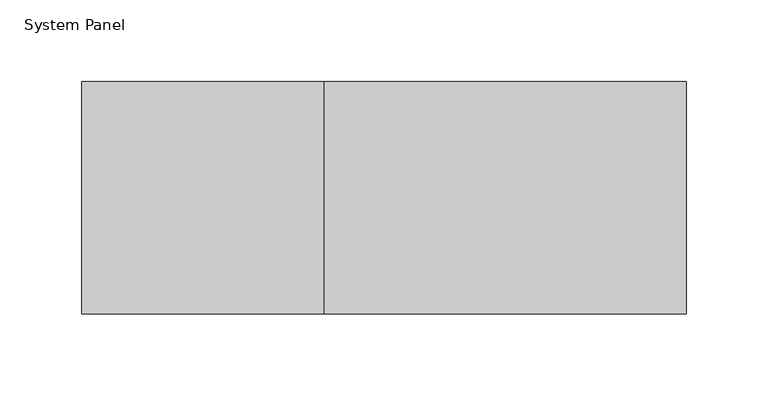
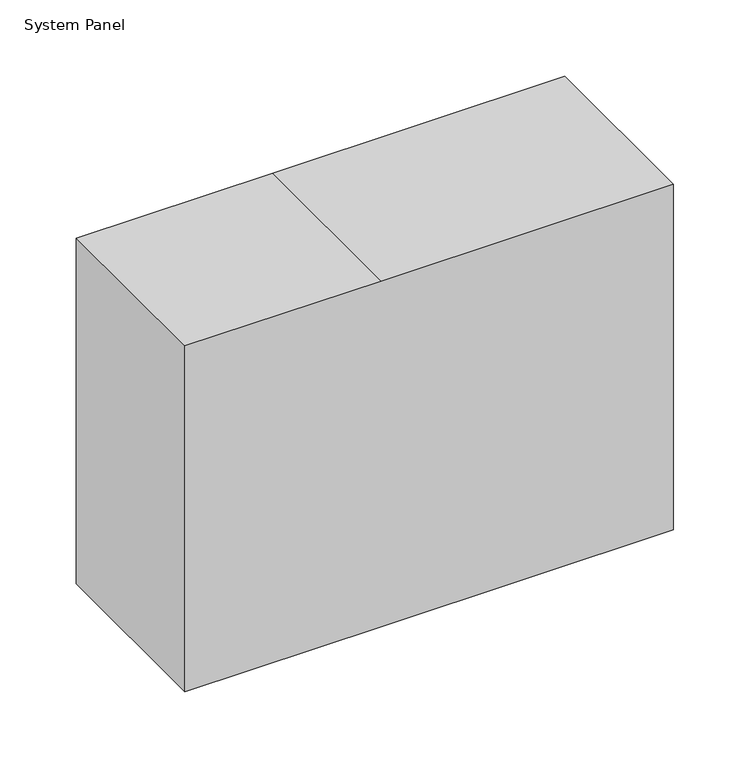
"""IFC4 building model written with IfcOpenShell, lengths in millimetres: plate geometry, System Panel : NLRS_21_CWP_hsb-vulling minerale wol 142 _gen_rsf."""

import ifcopenshell
import ifcopenshell.guid

model = None  # the IFC model being written
_history = None  # IfcOwnerHistory: only IFC2X3 demands one
_inside = {}  # id of a spatial element -> (the spatial element, [elements in it])
_under = {}  # id of a project, library or spatial element -> (it, [spatial elements below it])
_declared = {}  # id of a project -> (the project, [libraries it declares])
_typed = {}  # id of a type object -> (the type object, [elements of that type])
_made_of = {}  # id of a material, layer set ... -> (it, [elements and type objects made of it])


def new_model(schema):
    """Start an empty IFC model of exactly this schema.

    Asked for "IFC4X3", IfcOpenShell would pick the latest addendum, in which some entities
    have other attributes; the version numbers below select the first issue.
    IFC2X3 requires an IfcOwnerHistory on every rooted entity: one is made here for all.
    """
    global model, _history
    if schema == "IFC4X3":
        model = ifcopenshell.file(schema_version=(4, 3, 0, 0))
    else:
        model = ifcopenshell.file(schema=schema)
    _inside.clear()
    _under.clear()
    _declared.clear()
    _typed.clear()
    _made_of.clear()
    _history = None
    if model.schema == "IFC2X3":
        org = make("IfcOrganization", Name="unknown")
        user = make(
            "IfcPersonAndOrganization",
            ThePerson=make("IfcPerson", FamilyName="unknown"),
            TheOrganization=org,
        )
        app = make(
            "IfcApplication",
            ApplicationDeveloper=org,
            Version="unknown",
            ApplicationFullName="unknown",
            ApplicationIdentifier="unknown",
        )
        _history = make(
            "IfcOwnerHistory",
            OwningUser=user,
            OwningApplication=app,
            ChangeAction="ADDED",
            CreationDate=0,
        )
    return model


def make(cls, **values):
    """One entity of the class cls with the attributes given. An attribute that is None is left unset."""
    return model.create_entity(
        cls, **{name: value for name, value in values.items() if value is not None}
    )


def rooted(cls, **values):
    """An entity with a GlobalId (a new one), such as an element, a storey or a relation."""
    return make(cls, GlobalId=ifcopenshell.guid.new(), OwnerHistory=_history, **values)


def si_unit(unit_type, name, prefix=None):
    """IfcSIUnit, for example si_unit("LENGTHUNIT", "METRE", prefix="MILLI")."""
    return make("IfcSIUnit", UnitType=unit_type, Prefix=prefix, Name=name)


def assignment(units):
    """IfcUnitAssignment: the units of a project."""
    return None if units is None else make("IfcUnitAssignment", Units=units)


def point(xyz):
    """IfcCartesianPoint."""
    return None if xyz is None else make("IfcCartesianPoint", Coordinates=xyz)


def direction(xyz):
    """IfcDirection."""
    return None if xyz is None else make("IfcDirection", DirectionRatios=xyz)


def frame(location, z_axis=None, x_axis=None):
    """IfcAxis2Placement3D, a coordinate frame: its origin and axes. An axis left out is left unset."""
    return make(
        "IfcAxis2Placement3D",
        Location=point(location),
        Axis=direction(z_axis),
        RefDirection=direction(x_axis),
    )


def origin():
    """The frame at (0, 0, 0) with its axes left unset."""
    return frame((0.0, 0.0, 0.0))


def place(relative_to, where):
    """IfcLocalPlacement: puts the frame where relative to a parent placement (None: the world)."""
    return make(
        "IfcLocalPlacement", PlacementRelTo=relative_to, RelativePlacement=where
    )


def context(
    kind, dimensions, precision=None, world=None, true_north=None, identifier=None
):
    """IfcGeometricRepresentationContext, for example the 3D "Model" context."""
    return make(
        "IfcGeometricRepresentationContext",
        ContextIdentifier=identifier,
        ContextType=kind,
        CoordinateSpaceDimension=dimensions,
        Precision=precision,
        WorldCoordinateSystem=world,
        TrueNorth=true_north,
    )


def project(units=None, contexts=None):
    """IfcProject with its units and contexts."""
    return rooted(
        "IfcProject",
        Name="project",
        RepresentationContexts=contexts,
        UnitsInContext=assignment(units),
    )


def spatial(cls, under=None, at=None, **own):
    """A site, building, storey or space (cls), placed at a placement, below another one or the project."""
    s = rooted(cls, ObjectPlacement=at, **own)
    if under is not None:
        _under.setdefault(under.id(), (under, []))[1].append(s)
    return s


def polyline(points):
    """IfcPolyline through the points."""
    return make("IfcPolyline", Points=[point(p) for p in points])


def outline(outer, holes=None, kind="AREA"):
    """IfcArbitraryClosedProfileDef: a profile drawn as a closed curve; with holes, ...WithVoids."""
    if holes is None:
        return make("IfcArbitraryClosedProfileDef", ProfileType=kind, OuterCurve=outer)
    return make(
        "IfcArbitraryProfileDefWithVoids",
        ProfileType=kind,
        OuterCurve=outer,
        InnerCurves=holes,
    )


def extrude(swept, where, along, depth):
    """IfcExtrudedAreaSolid: the profile swept, set in the frame where, extruded along a direction by depth."""
    return make(
        "IfcExtrudedAreaSolid",
        SweptArea=swept,
        Position=where,
        ExtrudedDirection=direction(along),
        Depth=depth,
    )


def shape(context_of_items, identifier, shape_type, items):
    """IfcShapeRepresentation: the items that make up one representation, for example the "Body"."""
    return make(
        "IfcShapeRepresentation",
        ContextOfItems=context_of_items,
        RepresentationIdentifier=identifier,
        RepresentationType=shape_type,
        Items=items,
    )


def source(mapping_origin, context_of_items, identifier, shape_type, items):
    """IfcRepresentationMap: a shape defined once, which mapped items show again and again."""
    return make(
        "IfcRepresentationMap",
        MappingOrigin=mapping_origin,
        MappedRepresentation=shape(context_of_items, identifier, shape_type, items),
    )


def transform(
    local_origin,
    x_axis=None,
    y_axis=None,
    z_axis=None,
    scale=None,
    scale2=None,
    scale3=None,
    uniform=True,
):
    """IfcCartesianTransformationOperator3D, or its non-uniform kind. x_axis, y_axis, z_axis: its Axis1, 2, 3."""
    if uniform:
        return make(
            "IfcCartesianTransformationOperator3D",
            Axis1=direction(x_axis),
            Axis2=direction(y_axis),
            LocalOrigin=point(local_origin),
            Scale=scale,
            Axis3=direction(z_axis),
        )
    return make(
        "IfcCartesianTransformationOperator3DnonUniform",
        Axis1=direction(x_axis),
        Axis2=direction(y_axis),
        LocalOrigin=point(local_origin),
        Scale=scale,
        Axis3=direction(z_axis),
        Scale2=scale2,
        Scale3=scale3,
    )


def mapped(mapping_source, mapping_target):
    """IfcMappedItem: shows the shape of a source again, moved by a transform."""
    return make(
        "IfcMappedItem", MappingSource=mapping_source, MappingTarget=mapping_target
    )


def made_of(thing, what):
    """Note that an element or type object is made of a material, layer set ...; save() writes the relation."""
    if what is not None:
        _made_of.setdefault(what.id(), (what, []))[1].append(thing)
    return thing


def element(
    cls,
    number,
    at=None,
    inside=None,
    cuts=None,
    type_object=None,
    material=None,
    context=None,
    identifier="Body",
    shape_type=None,
    held_by="IfcProductDefinitionShape",
    body=None,
    shapes=None,
    **own,
):
    """One element of the class cls, such as IfcWall. Its Tag is "e" and its number.

    at: its placement. inside: the storey or other place that contains it. cuts: it is an
    opening in that element (IfcRelVoidsElement). A single representation is given by context,
    identifier, shape_type and body (its items); several are given by shapes. held_by: the class
    of the entity that holds the representations. save() writes the other relations.
    """
    e = rooted(cls, Tag="e%d" % number, ObjectPlacement=at, **own)
    if body is not None:
        shapes = [shape(context, identifier, shape_type, body)]
    if shapes is not None:
        e.Representation = make(held_by, Representations=shapes)
    if inside is not None:
        _inside.setdefault(inside.id(), (inside, []))[1].append(e)
    if cuts is not None:
        rooted(
            "IfcRelVoidsElement", RelatingBuildingElement=cuts, RelatedOpeningElement=e
        )
    if type_object is not None:
        _typed.setdefault(type_object.id(), (type_object, []))[1].append(e)
    return made_of(e, material)


def aggregate(whole, parts):
    """IfcRelAggregates: a whole, such as a stair, and the parts it consists of."""
    return rooted("IfcRelAggregates", RelatingObject=whole, RelatedObjects=parts)


def save(model, path):
    """Write the relations noted so far, then the file.

    IfcRelAggregates (storeys below a building ...), IfcRelContainedInSpatialStructure (elements
    in a storey), IfcRelDefinesByType, IfcRelAssociatesMaterial and IfcRelDeclares: one each for
    every whole, place, type object, material and project.
    """
    for whole, parts in _under.values():
        aggregate(whole, parts)
    for where, things in _inside.values():
        rooted(
            "IfcRelContainedInSpatialStructure",
            RelatedElements=things,
            RelatingStructure=where,
        )
    for kind, things in _typed.values():
        rooted("IfcRelDefinesByType", RelatedObjects=things, RelatingType=kind)
    for what, things in _made_of.values():
        rooted("IfcRelAssociatesMaterial", RelatedObjects=things, RelatingMaterial=what)
    for by, libraries in _declared.values():
        rooted("IfcRelDeclares", RelatingContext=by, RelatedDefinitions=libraries)
    model.write(path)


def system_panel_c31e55ff(model_context):
    return source(origin(), model_context, "Body", "SweptSolid", [
        extrude(outline(polyline([(0.0, -184.5), (0.0, -36.3441061), (0.0, 184.5), (276.0, 184.5), (276.0, -36.3441061), (276.0, -184.5), (0.0, -184.5)])), frame((0.0, -71.0, 0.0), z_axis=(0.0, 1.0, 0.0), x_axis=(0.0, 0.0, 1.0)), (0.0, 0.0, 1.0), 142.0),
    ])


if __name__ == "__main__":
    model = new_model("IFC4")
    model_context = context("Model", 3, world=origin())
    ifc_project = project(units=[si_unit("LENGTHUNIT", "METRE", prefix="MILLI")], contexts=[model_context])
    site = spatial("IfcSite", under=ifc_project)
    building = spatial("IfcBuilding", under=site)
    placement = place(None, origin())
    system_panel_shape = system_panel_c31e55ff(model_context)
    element("IfcPlate", 1, ObjectType="System Panel : NLRS_21_CWP_hsb-vulling minerale wol 142 _gen_rsf", at=placement, inside=building, context=model_context, shape_type="MappedRepresentation", body=[
        mapped(system_panel_shape, transform((0.0, 0.0, 0.0), x_axis=(1.0, 0.0, 0.0), y_axis=(0.0, 1.0, 0.0), z_axis=(0.0, 0.0, 1.0))),
    ])
    save(model, "model.ifc")

# Revit data of these elements
# Type "System Panel : NLRS_21_CWP_hsb-vulling minerale wol 142 _gen_rsf"
#   Export Type to IFC As = "IfcWall"
#   Type IfcGUID = "07M7mRoiH1CR8m_RSKIwpC"
#   Assembly Code = "21.23"
# Element 1 (IfcPlate, "System Panel : NLRS_21_CWP_hsb-vulling minerale wol 142 _gen_rsf")
#   Materials on its faces: "NLRS_m1_isolatie minerale wol_gen_rsf"
# Materials
#   "NLRS_m1_isolatie minerale wol_gen_rsf": class "M - Anorganische materialen", colour RGB 200 200 140, transparency 0, Keynote = "m1", Manufacturer = "Revit Standards Foundation", URL = "www.revitstandards.org", Description = "isolatie minerale wol", Cost = 0
